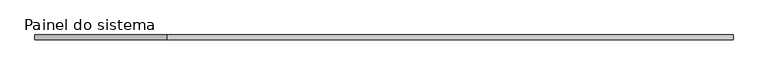
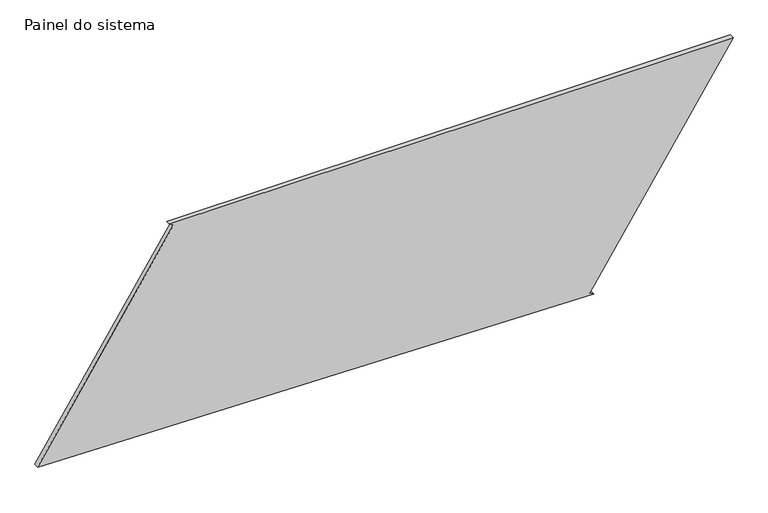
"""IFC4 building model written with IfcOpenShell, lengths in millimetres: plate geometry, Painel do sistema : Envidraçado."""

from ifc_helpers import new_model, si_unit, frame, origin, place, context, project, spatial, polyline, outline, extrude, source, transform, mapped, element, save


def painel_do_sistema_e86f411d(model_context):
    return source(origin(), model_context, "Body", "SweptSolid", [
        extrude(outline(polyline([(0.0, 1124.0976162), (13.6354654, 1103.1435215), (1200.2167846, 1875.2880014), (1200.2167846, -1164.2479209), (1186.5813192, -1143.2938263), (61.7003719, -1875.2880014), (0.0, 1124.0976162)])), frame((0.0, 24.5, 0.0), z_axis=(0.0, 1.0, 0.0), x_axis=(0.0, 0.0, 1.0)), (0.0, 0.0, 1.0), 25.0),
    ])


if __name__ == "__main__":
    model = new_model("IFC4")
    model_context = context("Model", 3, world=origin())
    ifc_project = project(units=[si_unit("LENGTHUNIT", "METRE", prefix="MILLI")], contexts=[model_context])
    site = spatial("IfcSite", under=ifc_project)
    building = spatial("IfcBuilding", under=site)
    placement = place(None, origin())
    painel_do_sistema_shape = painel_do_sistema_e86f411d(model_context)
    element("IfcPlate", 1, ObjectType="Painel do sistema : Envidraçado", at=placement, inside=building, context=model_context, shape_type="MappedRepresentation", body=[
        mapped(painel_do_sistema_shape, transform((0.0, 0.0, 0.0), x_axis=(1.0, 0.0, 0.0), y_axis=(0.0, 1.0, 0.0), z_axis=(0.0, 0.0, 1.0))),
    ])
    save(model, "model.ifc")

# Revit data of these elements
# Type "Painel do sistema : Envidraçado"
#   Construction Type Id = "GSP4R"
#   Analytic Construction = "Vidraça única Pilkington 1/8 pol"
#   Visual Light Transmittance = 0.9
#   Solar Heat Gain Coefficient = 0.86
#   Heat Transfer Coefficient (U) = 6.7069 W/(m²·K)
# Element 1 (IfcPlate, "Painel do sistema : Envidraçado")
#   Materials on its faces: "Vidro"
# Materials
#   "Vidro": class "Vidro", colour RGB 0 128 192, transparency 0.9, Description = "Vidro de sílica", Cost = 0
